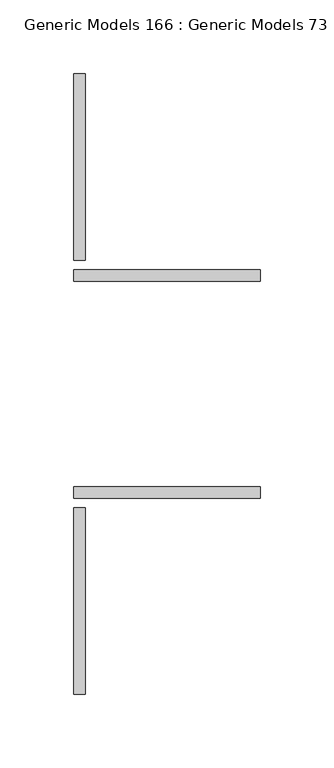
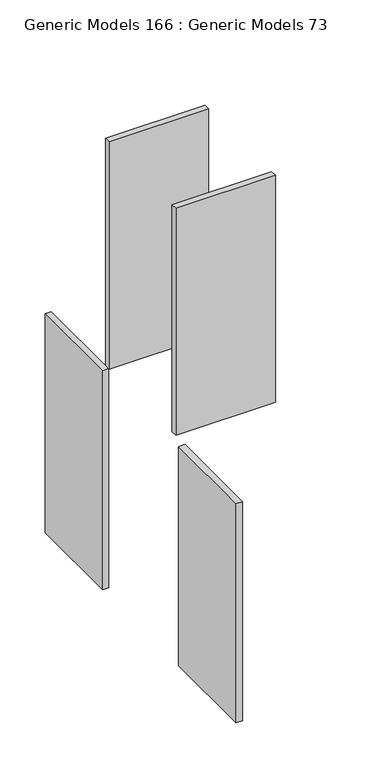
"""IFC4 building model written with IfcOpenShell, lengths in millimetres: proxy geometry, Generic Models 166 : Generic Models 73."""

from ifc_helpers import new_model, si_unit, frame, origin, place, context, project, spatial, polyline, outline, extrude, source, transform, mapped, element, save


def generic_models_166_generic_models_73_e2e018fc(model_context):
    return source(origin(), model_context, "Body", "SweptSolid", [
        extrude(outline(polyline([(31923.0340778, 30690.2031612), (31930.9715778, 30690.2031612), (31930.9715778, 30563.2031612), (31923.0340778, 30563.2031612), (31923.0340778, 30690.2031612)])), frame((0.0, 0.0, 271490.7765953), z_axis=(0.0, 0.0, 1.0), x_axis=(1.0, 0.0, 0.0)), (0.0, 0.0, 1.0), 295.5734047),
        extrude(outline(polyline([(31923.0340778, 30985.4781612), (31930.9715778, 30985.4781612), (31930.9715778, 30858.4781612), (31923.0340778, 30858.4781612), (31923.0340778, 30985.4781612)])), frame((0.0, 0.0, 271490.7765953), z_axis=(0.0, 0.0, 1.0), x_axis=(1.0, 0.0, 0.0)), (0.0, 0.0, 1.0), 295.5734047),
        extrude(outline(polyline([(32050.0340778, 30852.1281612), (32050.0340778, 30844.1906612), (31923.0340778, 30844.1906612), (31923.0340778, 30852.1281612), (32050.0340778, 30852.1281612)])), frame((0.0, 0.0, 271797.4625), z_axis=(0.0, 0.0, 1.0), x_axis=(1.0, 0.0, 0.0)), (0.0, 0.0, 1.0), 306.5595065),
        extrude(outline(polyline([(32050.0340778, 30704.4906612), (32050.0340778, 30696.5531612), (31923.0340778, 30696.5531612), (31923.0340778, 30704.4906612), (32050.0340778, 30704.4906612)])), frame((0.0, 0.0, 271797.4625), z_axis=(0.0, 0.0, 1.0), x_axis=(1.0, 0.0, 0.0)), (0.0, 0.0, 1.0), 306.5595065),
    ])


if __name__ == "__main__":
    model = new_model("IFC4")
    model_context = context("Model", 3, world=origin())
    ifc_project = project(units=[si_unit("LENGTHUNIT", "METRE", prefix="MILLI")], contexts=[model_context])
    site = spatial("IfcSite", under=ifc_project)
    building = spatial("IfcBuilding", under=site)
    placement = place(None, origin())
    generic_models_166_generic_models_73_shape = generic_models_166_generic_models_73_e2e018fc(model_context)
    element("IfcBuildingElementProxy", 1, Name="Generic Models 166 : Generic Models 73", ObjectType="Generic Models 166 : Generic Models 73", at=placement, inside=building, context=model_context, shape_type="MappedRepresentation", body=[
        mapped(generic_models_166_generic_models_73_shape, transform((0.0, 0.0, 0.0), x_axis=(1.0, 0.0, 0.0), y_axis=(0.0, 1.0, 0.0), z_axis=(0.0, 0.0, 1.0))),
    ])
    save(model, "model.ifc")

# Revit data of these elements
# Element 1 (IfcBuildingElementProxy, "Generic Models 166 : Generic Models 73")
#   Materials on its faces: "5/16\" THICK GALV. STEEL PLATE", "5/16 THICK GALV. SADDLE"
# Materials
#   "5/16\" THICK GALV. STEEL PLATE": class "Metal", colour RGB 199 199 199, transparency 0, Description = "Carbon steel", Cost = 0
#   "5/16 THICK GALV. SADDLE": class "Metal", colour RGB 199 199 199, transparency 0, Description = "Carbon steel", Cost = 0
